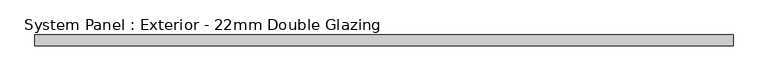
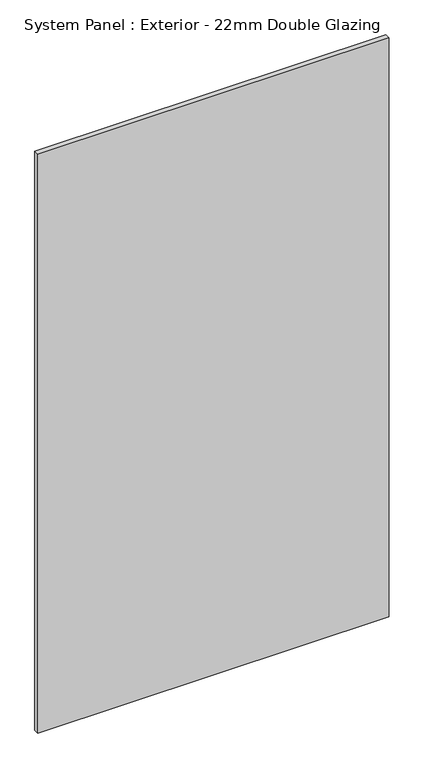
"""IFC4 building model written with IfcOpenShell, lengths in millimetres: plate geometry, System Panel : Exterior - 22mm Double Glazing."""

from ifc_helpers import new_model, si_unit, origin, origin_with_axes, place, context, project, spatial, polyline, outline, extrude, source, transform, mapped, element, save


def system_panel_exterior_22mm_double_glazing_aa15faa2(model_context):
    return source(origin(), model_context, "Body", "SweptSolid", [
        extrude(outline(polyline([(724.9999999, 15.0), (-724.9999999, 15.0), (-724.9999999, 37.0), (724.9999999, 37.0), (724.9999999, 15.0)])), origin_with_axes(), (0.0, 0.0, 1.0), 2525.0),
    ])


if __name__ == "__main__":
    model = new_model("IFC4")
    model_context = context("Model", 3, world=origin())
    ifc_project = project(units=[si_unit("LENGTHUNIT", "METRE", prefix="MILLI")], contexts=[model_context])
    site = spatial("IfcSite", under=ifc_project)
    building = spatial("IfcBuilding", under=site)
    placement = place(None, origin())
    system_panel_exterior_22mm_double_glazing_shape = system_panel_exterior_22mm_double_glazing_aa15faa2(model_context)
    element("IfcPlate", 1, ObjectType="System Panel : Exterior - 22mm Double Glazing", at=placement, inside=building, context=model_context, shape_type="MappedRepresentation", body=[
        mapped(system_panel_exterior_22mm_double_glazing_shape, transform((0.0, 0.0, 0.0), x_axis=(1.0, 0.0, 0.0), y_axis=(0.0, 1.0, 0.0), z_axis=(0.0, 0.0, 1.0))),
    ])
    save(model, "model.ifc")

# Revit data of these elements
# Element 1 (IfcPlate, "System Panel : Exterior - 22mm Double Glazing")
#   Materials on its faces: "Glass"
# Materials
#   "Glass": class "Glass", colour RGB 180 200 255, transparency 0.75, Description = "Generisk glas", Cost = 0
